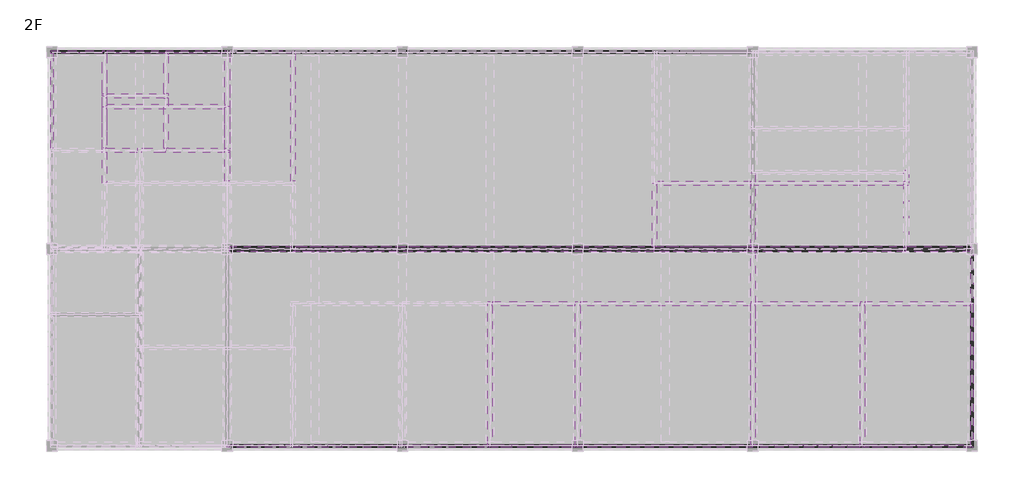
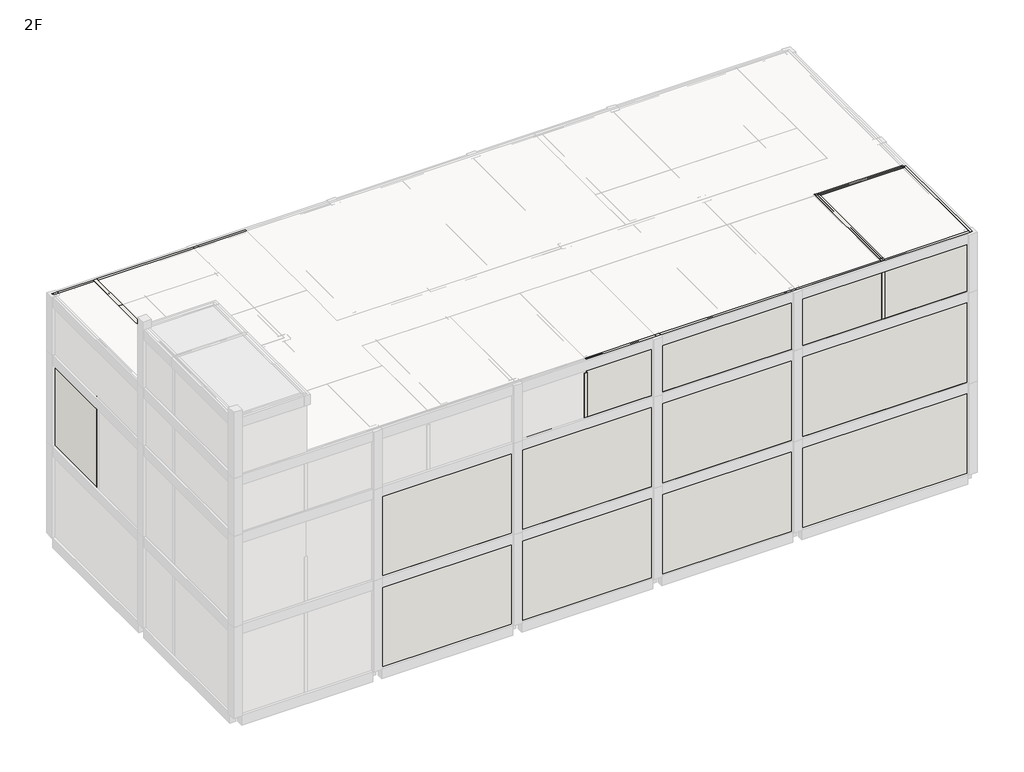
# One storey, part 2 of 7: 53 walls.
"""IFC4 building model written with IfcOpenShell, lengths in millimetres."""

from ifc_helpers import new_model, si_unit, frame, origin, place, context, project, spatial, polyline, outline, extrude, faceted_brep, element, save

model = new_model("IFC4")

# Units and contexts
model_context = context("Model", 3, world=origin())
ifc_project = project(units=[si_unit("LENGTHUNIT", "METRE", prefix="MILLI")], contexts=[model_context])

# Site, building, storey
site = spatial("IfcSite", under=ifc_project)
building = spatial("IfcBuilding", under=site)
storey = spatial("IfcBuildingStorey", under=building, Name="2F", Elevation=3500.0)

# Walls
placement = place(None, origin())
element("IfcWall", 1, ObjectType="WA211_Exterior-Cement Brick-90mm", at=placement, inside=storey, context=model_context, shape_type="Brep", body=[
    faceted_brep([(45402.6521483, 181866.8614395, 3500.0), (45516.6521483, 181866.8614395, 3500.0), (77352.6521483, 181866.8614395, 3500.0), (77352.6521483, 181866.8614395, 9000.0), (45516.6521483, 181866.8614395, 9000.0), (45402.6521483, 181866.8614395, 9000.0), (45402.6521483, 181980.8614395, 3500.0), (45402.6521483, 181980.8614395, 9000.0), (77352.6521483, 181980.8614395, 9000.0), (77352.6521483, 181980.8614395, 3500.0)], [[[0, 1, 2, 3, 4, 5]], [[6, 7, 8, 9]], [[2, 1, 0, 6, 9]], [[5, 4, 3, 8, 7]], [[0, 5, 7, 6]], [[3, 2, 9, 8]]]),
])
element("IfcWall", 2, ObjectType="WA211_Exterior-Cement Brick-90mm", at=placement, inside=storey, context=model_context, shape_type="SweptSolid", body=[
    extrude(outline(polyline([(53566.6521483, 163980.8614395), (87402.6521483, 163980.8614395), (87402.6521483, 163866.8614395), (53566.6521483, 163866.8614395), (53566.6521483, 163980.8614395)])), frame((0.0, 0.0, 3500.0), z_axis=(0.0, 0.0, 1.0), x_axis=(1.0, 0.0, 0.0)), (0.0, 0.0, 1.0), 5500.0),
])
element("IfcWall", 3, ObjectType="WA211_Exterior-Cement Brick-90mm", at=placement, inside=storey, context=model_context, shape_type="Brep", body=[
    faceted_brep([(87402.6521483, 172923.8614395, 3500.0), (87402.6521483, 172816.8614395, 3500.0), (87402.6521483, 163980.8614395, 3500.0), (87402.6521483, 163866.8614395, 3500.0), (87402.6521483, 163866.8614395, 9000.0), (87402.6521483, 163980.8614395, 9000.0), (87402.6521483, 172816.8614395, 9000.0), (87402.6521483, 172923.8614395, 9000.0), (87516.6521483, 172923.8614395, 3500.0), (87516.6521483, 172923.8614395, 9000.0), (87516.6521483, 163866.8614395, 9000.0), (87516.6521483, 163866.8614395, 3500.0)], [[[0, 1, 2, 3, 4, 5, 6, 7]], [[8, 9, 10, 11]], [[3, 2, 1, 0, 8, 11]], [[7, 6, 5, 4, 10, 9]], [[0, 7, 9, 8]], [[4, 3, 11, 10]]]),
])
element("IfcWall", 4, ObjectType="WA211_Exterior-Cement Brick-90mm", at=placement, inside=storey, context=model_context, shape_type="Brep", body=[
    faceted_brep([(77459.6521483, 163980.8614395, 9000.0), (77352.6521483, 163980.8614395, 9000.0), (53566.6521483, 163980.8614395, 9000.0), (53566.6521483, 163980.8614395, 12000.0), (53459.6521483, 163980.8614395, 12000.0), (53459.6521483, 163980.8614395, 14500.0), (77352.6521483, 163980.8614395, 14500.0), (77459.6521483, 163980.8614395, 14500.0), (77459.6521483, 163866.8614395, 9000.0), (77459.6521483, 163866.8614395, 14500.0), (53459.6521483, 163866.8614395, 14500.0), (53459.6521483, 163866.8614395, 12000.0), (53566.6521483, 163866.8614395, 12000.0), (53566.6521483, 163866.8614395, 9000.0)], [[[0, 1, 2, 3, 4, 5, 6, 7]], [[8, 9, 10, 11, 12, 13]], [[2, 1, 0, 8, 13]], [[7, 6, 5, 10, 9]], [[0, 7, 9, 8]], [[5, 4, 11, 10]], [[11, 4, 3, 12]], [[3, 2, 13, 12]]]),
])
element("IfcWall", 5, ObjectType="WA211_Exterior-Cement Brick-90mm", at=placement, inside=storey, context=model_context, shape_type="Brep", body=[
    faceted_brep([(87402.6521483, 163980.8614395, 9000.0), (77566.6521483, 163980.8614395, 9000.0), (77459.6521483, 163980.8614395, 9000.0), (77459.6521483, 163980.8614395, 14500.0), (77566.6521483, 163980.8614395, 14500.0), (87402.6521483, 163980.8614395, 14500.0), (87402.6521483, 163866.8614395, 9000.0), (87402.6521483, 163866.8614395, 14500.0), (77459.6521483, 163866.8614395, 14500.0), (77459.6521483, 163866.8614395, 9000.0)], [[[0, 1, 2, 3, 4, 5]], [[6, 7, 8, 9]], [[2, 1, 0, 6, 9]], [[3, 2, 9, 8]], [[5, 4, 3, 8, 7]], [[0, 5, 7, 6]]]),
])
element("IfcWall", 6, ObjectType="WA211_Exterior-Cement Brick-90mm", at=placement, inside=storey, context=model_context, shape_type="Brep", body=[
    faceted_brep([(87402.6521483, 172923.8614395, 9000.0), (87402.6521483, 172816.8614395, 9000.0), (87402.6521483, 163980.8614395, 9000.0), (87402.6521483, 163866.8614395, 9000.0), (87402.6521483, 163866.8614395, 14500.0), (87402.6521483, 163980.8614395, 14500.0), (87402.6521483, 172816.8614395, 14500.0), (87402.6521483, 172923.8614395, 14500.0), (87516.6521483, 172923.8614395, 9000.0), (87516.6521483, 172923.8614395, 14500.0), (87516.6521483, 163866.8614395, 14500.0), (87516.6521483, 163866.8614395, 9000.0)], [[[0, 1, 2, 3, 4, 5, 6, 7]], [[8, 9, 10, 11]], [[3, 2, 1, 0, 8, 11]], [[7, 6, 5, 4, 10, 9]], [[0, 7, 9, 8]], [[4, 3, 11, 10]]]),
])
element("IfcWall", 7, ObjectType="WA211_Exterior-Cement Brick-90mm", at=placement, inside=storey, context=model_context, shape_type="SweptSolid", body=[
    extrude(outline(polyline([(45516.6521483, 181866.8614395), (45516.6521483, 177530.8614395), (45402.6521483, 177530.8614395), (45402.6521483, 181866.8614395), (45516.6521483, 181866.8614395)])), frame((0.0, 0.0, 9000.0), z_axis=(0.0, 0.0, 1.0), x_axis=(1.0, 0.0, 0.0)), (0.0, 0.0, 1.0), 5500.0),
])
element("IfcWall", 8, ObjectType="WA211_Exterior-Cement Brick-90mm", at=placement, inside=storey, context=model_context, shape_type="Brep", body=[
    faceted_brep([(45402.6521483, 181866.8614395, 9000.0), (45516.6521483, 181866.8614395, 9000.0), (47752.6521483, 181866.8614395, 9000.0), (47752.6521483, 181866.8614395, 14500.0), (45516.6521483, 181866.8614395, 14500.0), (45402.6521483, 181866.8614395, 14500.0), (45402.6521483, 181980.8614395, 9000.0), (45402.6521483, 181980.8614395, 14500.0), (47752.6521483, 181980.8614395, 14500.0), (47752.6521483, 181980.8614395, 9000.0)], [[[0, 1, 2, 3, 4, 5]], [[6, 7, 8, 9]], [[2, 1, 0, 6, 9]], [[5, 4, 3, 8, 7]], [[0, 5, 7, 6]], [[3, 2, 9, 8]]]),
])
element("IfcWall", 9, ObjectType="WA211_Exterior-Cement Brick-90mm", at=placement, inside=storey, context=model_context, shape_type="Brep", body=[
    faceted_brep([(50659.6521483, 181866.8614395, 14500.0), (50659.6521483, 181866.8614395, 9000.0), (50766.6521483, 181866.8614395, 9000.0), (53352.6521483, 181866.8614395, 9000.0), (53352.6521483, 181866.8614395, 12400.0), (53459.6521483, 181866.8614395, 12400.0), (53459.6521483, 181866.8614395, 14500.0), (50659.6521483, 181980.8614395, 9000.0), (50659.6521483, 181980.8614395, 14500.0), (53459.6521483, 181980.8614395, 14500.0), (53459.6521483, 181980.8614395, 12400.0), (53352.6521483, 181980.8614395, 12400.0), (53352.6521483, 181980.8614395, 9000.0)], [[[0, 1, 2, 3, 4, 5, 6]], [[7, 8, 9, 10, 11, 12]], [[3, 2, 1, 7, 12]], [[0, 6, 9, 8]], [[6, 5, 10, 9]], [[10, 5, 4, 11]], [[4, 3, 12, 11]], [[0, 8, 7, 1]]]),
])
element("IfcWall", 10, ObjectType="WA211_Exterior-Cement Brick-90mm", at=placement, inside=storey, context=model_context, shape_type="Brep", body=[
    faceted_brep([(47966.6521483, 181866.8614395, 9000.0), (50552.6521483, 181866.8614395, 9000.0), (50659.6521483, 181866.8614395, 9000.0), (50659.6521483, 181866.8614395, 14500.0), (47966.6521483, 181866.8614395, 14500.0), (47966.6521483, 181980.8614395, 9000.0), (47966.6521483, 181980.8614395, 14500.0), (50659.6521483, 181980.8614395, 14500.0), (50659.6521483, 181980.8614395, 9000.0)], [[[0, 1, 2, 3, 4]], [[5, 6, 7, 8]], [[2, 1, 0, 5, 8]], [[4, 3, 7, 6]], [[0, 4, 6, 5]], [[2, 8, 7, 3]]]),
])
element("IfcWall", 11, ObjectType="WA211_Exterior-Cement Brick-90mm", at=placement, inside=storey, context=model_context, shape_type="SweptSolid", body=[
    extrude(outline(polyline([(14500.0, 69352.6521483), (17200.0, 69352.6521483), (17200.0, 69459.6521483), (18000.0, 69459.6521483), (18000.0, 65459.6521483), (17200.0, 65459.6521483), (17200.0, 65566.6521483), (14500.0, 65566.6521483), (14500.0, 69352.6521483)])), frame((0.0, 163866.8614395, 0.0), z_axis=(0.0, 1.0, 0.0), x_axis=(0.0, 0.0, 1.0)), (0.0, 0.0, 1.0), 114.0),
])
element("IfcWall", 12, ObjectType="WA211_Exterior-Cement Brick-90mm", at=placement, inside=storey, context=model_context, shape_type="Brep", body=[
    faceted_brep([(77459.6521483, 163980.8614395, 18000.0), (77459.6521483, 163980.8614395, 14500.0), (77352.6521483, 163980.8614395, 14500.0), (69566.6521483, 163980.8614395, 14500.0), (69566.6521483, 163980.8614395, 17200.0), (69459.6521483, 163980.8614395, 17200.0), (69459.6521483, 163980.8614395, 18000.0), (77459.6521483, 163866.8614395, 14500.0), (77459.6521483, 163866.8614395, 18000.0), (69459.6521483, 163866.8614395, 18000.0), (69459.6521483, 163866.8614395, 17200.0), (69566.6521483, 163866.8614395, 17200.0), (69566.6521483, 163866.8614395, 14500.0)], [[[0, 1, 2, 3, 4, 5, 6]], [[7, 8, 9, 10, 11, 12]], [[3, 2, 1, 7, 12]], [[0, 6, 9, 8]], [[6, 5, 10, 9]], [[10, 5, 4, 11]], [[4, 3, 12, 11]], [[0, 8, 7, 1]]]),
])
element("IfcWall", 13, ObjectType="WA211_Exterior-Cement Brick-90mm", at=placement, inside=storey, context=model_context, shape_type="Brep", body=[
    faceted_brep([(82352.6521483, 163980.8614395, 14500.0), (77566.6521483, 163980.8614395, 14500.0), (77459.6521483, 163980.8614395, 14500.0), (77459.6521483, 163980.8614395, 18000.0), (82352.6521483, 163980.8614395, 18000.0), (82352.6521483, 163866.8614395, 14500.0), (82352.6521483, 163866.8614395, 18000.0), (77459.6521483, 163866.8614395, 18000.0), (77459.6521483, 163866.8614395, 14500.0)], [[[0, 1, 2, 3, 4]], [[5, 6, 7, 8]], [[2, 1, 0, 5, 8]], [[4, 3, 7, 6]], [[2, 8, 7, 3]], [[0, 4, 6, 5]]]),
])
element("IfcWall", 14, ObjectType="WA211_Exterior-Cement Brick-90mm", at=placement, inside=storey, context=model_context, shape_type="SweptSolid", body=[
    extrude(outline(polyline([(82566.6521483, 163980.8614395), (87402.6521483, 163980.8614395), (87402.6521483, 163866.8614395), (82566.6521483, 163866.8614395), (82566.6521483, 163980.8614395)])), frame((0.0, 0.0, 14500.0), z_axis=(0.0, 0.0, 1.0), x_axis=(1.0, 0.0, 0.0)), (0.0, 0.0, 1.0), 3500.0),
])
element("IfcWall", 15, ObjectType="WA211_Exterior-Cement Brick-90mm", at=placement, inside=storey, context=model_context, shape_type="Brep", body=[
    faceted_brep([(87402.6521483, 170423.8614395, 14500.0), (87402.6521483, 170316.8614395, 14500.0), (87402.6521483, 163980.8614395, 14500.0), (87402.6521483, 163866.8614395, 14500.0), (87402.6521483, 163866.8614395, 18000.0), (87402.6521483, 163980.8614395, 18000.0), (87402.6521483, 170316.8614395, 18000.0), (87402.6521483, 170423.8614395, 18000.0), (87516.6521483, 170423.8614395, 14500.0), (87516.6521483, 170423.8614395, 18000.0), (87516.6521483, 163866.8614395, 18000.0), (87516.6521483, 163866.8614395, 14500.0)], [[[0, 1, 2, 3, 4, 5, 6, 7]], [[8, 9, 10, 11]], [[3, 2, 1, 0, 8, 11]], [[7, 6, 5, 4, 10, 9]], [[0, 7, 9, 8]], [[4, 3, 11, 10]]]),
])
element("IfcWall", 16, ObjectType="WA211_Exterior-Cement Brick-90mm", at=placement, inside=storey, context=model_context, shape_type="SweptSolid", body=[
    extrude(outline(polyline([(14500.0, 47966.6521483), (14500.0, 53352.6521483), (17200.0, 53352.6521483), (17200.0, 53459.6521483), (18000.0, 53459.6521483), (18000.0, 47966.6521483), (14500.0, 47966.6521483)])), frame((0.0, 181866.8614395, 0.0), z_axis=(0.0, 1.0, 0.0), x_axis=(0.0, 0.0, 1.0)), (0.0, 0.0, 1.0), 114.0),
])
element("IfcWall", 17, ObjectType="WA211_Exterior-Cement Brick-90mm", at=placement, inside=storey, context=model_context, shape_type="SweptSolid", body=[
    extrude(outline(polyline([(14500.0, 53566.6521483), (14500.0, 56352.6521483), (17200.0, 56352.6521483), (17200.0, 56459.6521483), (18000.0, 56459.6521483), (18000.0, 53459.6521483), (17200.0, 53459.6521483), (17200.0, 53566.6521483), (14500.0, 53566.6521483)])), frame((0.0, 181866.8614395, 0.0), z_axis=(0.0, 1.0, 0.0), x_axis=(0.0, 0.0, 1.0)), (0.0, 0.0, 1.0), 114.0),
])
element("IfcWall", 18, ObjectType="WA211_Exterior-Cement Brick-90mm", at=placement, inside=storey, context=model_context, shape_type="Brep", body=[
    faceted_brep([(45402.6521483, 181866.8614395, 14500.0), (45516.6521483, 181866.8614395, 14500.0), (47752.6521483, 181866.8614395, 14500.0), (47752.6521483, 181866.8614395, 18000.0), (45516.6521483, 181866.8614395, 18000.0), (45402.6521483, 181866.8614395, 18000.0), (45402.6521483, 181980.8614395, 14500.0), (45402.6521483, 181980.8614395, 18000.0), (47752.6521483, 181980.8614395, 18000.0), (47752.6521483, 181980.8614395, 14500.0)], [[[0, 1, 2, 3, 4, 5]], [[6, 7, 8, 9]], [[2, 1, 0, 6, 9]], [[5, 4, 3, 8, 7]], [[3, 2, 9, 8]], [[0, 5, 7, 6]]]),
])
element("IfcWall", 19, ObjectType="WA221_Interior-Cement Block-190mm", at=placement, inside=storey, context=model_context, shape_type="SweptSolid", body=[
    extrude(outline(polyline([(53566.6521483, 173030.8614395), (77352.6521483, 173030.8614395), (77352.6521483, 172816.8614395), (53566.6521483, 172816.8614395), (53566.6521483, 173030.8614395)])), frame((0.0, 0.0, 3500.0), z_axis=(0.0, 0.0, 1.0), x_axis=(1.0, 0.0, 0.0)), (0.0, 0.0, 1.0), 5500.0),
])
element("IfcWall", 20, ObjectType="WA221_Interior-Cement Block-190mm", at=placement, inside=storey, context=model_context, shape_type="Brep", body=[
    faceted_brep([(77566.6521483, 172816.8614395, 3500.0), (87402.6521483, 172816.8614395, 3500.0), (87402.6521483, 172816.8614395, 9000.0), (77566.6521483, 172816.8614395, 9000.0), (77566.6521483, 173030.8614395, 3500.0), (77566.6521483, 173030.8614395, 9000.0), (87402.6521483, 173030.8614395, 9000.0), (87402.6521483, 173030.8614395, 3500.0), (87402.6521483, 172923.8614395, 3500.0), (87402.6521483, 172923.8614395, 9000.0)], [[[0, 1, 2, 3]], [[4, 5, 6, 7]], [[1, 0, 4, 7, 8]], [[3, 2, 9, 6, 5]], [[0, 3, 5, 4]], [[2, 1, 8, 7, 6, 9]]]),
])
element("IfcWall", 21, ObjectType="WA221_Interior-Cement Block-190mm", at=placement, inside=storey, context=model_context, shape_type="Brep", body=[
    faceted_brep([(77459.6521483, 173030.8614395, 9000.0), (77352.6521483, 173030.8614395, 9000.0), (53566.6521483, 173030.8614395, 9000.0), (53566.6521483, 173030.8614395, 12400.0), (77352.6521483, 173030.8614395, 12400.0), (77459.6521483, 173030.8614395, 12400.0), (77459.6521483, 172816.8614395, 9000.0), (77459.6521483, 172816.8614395, 12400.0), (77352.6521483, 172816.8614395, 12400.0), (53566.6521483, 172816.8614395, 12400.0), (53566.6521483, 172816.8614395, 12000.0), (53566.6521483, 172816.8614395, 9000.0), (77352.6521483, 172816.8614395, 9000.0), (53566.6521483, 172923.8614395, 9000.0)], [[[0, 1, 2, 3, 4, 5]], [[6, 7, 8, 9, 10, 11, 12]], [[2, 1, 0, 6, 12, 11, 13]], [[5, 4, 3, 9, 8, 7]], [[0, 5, 7, 6]], [[2, 13, 11, 10, 9, 3]]]),
])
element("IfcWall", 22, ObjectType="WA221_Interior-Cement Block-190mm", at=placement, inside=storey, context=model_context, shape_type="Brep", body=[
    faceted_brep([(77352.6521483, 176316.8614395, 9000.0), (77352.6521483, 173030.8614395, 9000.0), (77352.6521483, 173030.8614395, 12400.0), (77352.6521483, 176423.8614395, 12400.0), (77352.6521483, 176423.8614395, 11700.0), (77352.6521483, 176316.8614395, 11700.0), (77566.6521483, 176316.8614395, 9000.0), (77566.6521483, 176316.8614395, 11700.0), (77566.6521483, 176423.8614395, 11700.0), (77566.6521483, 176423.8614395, 12400.0), (77566.6521483, 173030.8614395, 12400.0), (77566.6521483, 173030.8614395, 9000.0), (77459.6521483, 173030.8614395, 9000.0), (77459.6521483, 173030.8614395, 12400.0)], [[[0, 1, 2, 3, 4, 5]], [[6, 7, 8, 9, 10, 11]], [[1, 0, 6, 11, 12]], [[3, 2, 13, 10, 9]], [[2, 1, 12, 11, 10, 13]], [[4, 3, 9, 8]], [[4, 8, 7, 5]], [[0, 5, 7, 6]]]),
])
element("IfcWall", 23, ObjectType="WA221_Interior-Cement Block-190mm", at=placement, inside=storey, context=model_context, shape_type="Brep", body=[
    faceted_brep([(53566.6521483, 177530.8614395, 9000.0), (53566.6521483, 181866.8614395, 9000.0), (53566.6521483, 181980.8614395, 9000.0), (53566.6521483, 181980.8614395, 12400.0), (53566.6521483, 181866.8614395, 12400.0), (53566.6521483, 177423.8614395, 12400.0), (53566.6521483, 177423.8614395, 11700.0), (53566.6521483, 177530.8614395, 11700.0), (53352.6521483, 177530.8614395, 9000.0), (53352.6521483, 177530.8614395, 11700.0), (53352.6521483, 177423.8614395, 11700.0), (53352.6521483, 177423.8614395, 12400.0), (53352.6521483, 181866.8614395, 12400.0), (53352.6521483, 181980.8614395, 12400.0), (53352.6521483, 181980.8614395, 9000.0), (53352.6521483, 181866.8614395, 9000.0), (53459.6521483, 181980.8614395, 12400.0)], [[[0, 1, 2, 3, 4, 5, 6, 7]], [[8, 9, 10, 11, 12, 13, 14, 15]], [[2, 1, 0, 8, 15, 14]], [[5, 4, 3, 16, 13, 12, 11]], [[3, 2, 14, 13, 16]], [[6, 5, 11, 10]], [[6, 10, 9, 7]], [[0, 7, 9, 8]]]),
])
element("IfcWall", 24, ObjectType="WA221_Interior-Cement Block-190mm", at=placement, inside=storey, context=model_context, shape_type="Brep", body=[
    faceted_brep([(77566.6521483, 163980.8614395, 9000.0), (77566.6521483, 172816.8614395, 9000.0), (77566.6521483, 172816.8614395, 14500.0), (77566.6521483, 163980.8614395, 14500.0), (77352.6521483, 163980.8614395, 9000.0), (77352.6521483, 163980.8614395, 14500.0), (77352.6521483, 172816.8614395, 14500.0), (77352.6521483, 172816.8614395, 12400.0), (77352.6521483, 172816.8614395, 9000.0), (77459.6521483, 163980.8614395, 9000.0), (77459.6521483, 172816.8614395, 9000.0), (77459.6521483, 163980.8614395, 14500.0)], [[[0, 1, 2, 3]], [[4, 5, 6, 7, 8]], [[1, 0, 9, 4, 8, 10]], [[3, 2, 6, 5, 11]], [[1, 10, 8, 7, 6, 2]], [[0, 3, 11, 5, 4, 9]]]),
])
element("IfcWall", 25, ObjectType="WA221_Interior-Cement Block-190mm", at=placement, inside=storey, context=model_context, shape_type="Brep", body=[
    faceted_brep([(77459.6521483, 172816.8614395, 9000.0), (77566.6521483, 172816.8614395, 9000.0), (84459.6521483, 172816.8614395, 9000.0), (84459.6521483, 172816.8614395, 14500.0), (77566.6521483, 172816.8614395, 14500.0), (77352.6521483, 172816.8614395, 14500.0), (77352.6521483, 172816.8614395, 12400.0), (77459.6521483, 172816.8614395, 12400.0), (77459.6521483, 173030.8614395, 9000.0), (77459.6521483, 173030.8614395, 12400.0), (77352.6521483, 173030.8614395, 12400.0), (77352.6521483, 173030.8614395, 14500.0), (84459.6521483, 173030.8614395, 14500.0), (84459.6521483, 173030.8614395, 9000.0), (84352.6521483, 173030.8614395, 9000.0), (77566.6521483, 173030.8614395, 9000.0)], [[[0, 1, 2, 3, 4, 5, 6, 7]], [[8, 9, 10, 11, 12, 13, 14, 15]], [[2, 1, 0, 8, 15, 14, 13]], [[5, 4, 3, 12, 11]], [[0, 7, 9, 8]], [[6, 10, 9, 7]], [[6, 5, 11, 10]], [[2, 13, 12, 3]]]),
])
element("IfcWall", 26, ObjectType="WA221_Interior-Cement Block-190mm", at=placement, inside=storey, context=model_context, shape_type="Brep", body=[
    faceted_brep([(84459.6521483, 172816.8614395, 14500.0), (84459.6521483, 172816.8614395, 9000.0), (87402.6521483, 172816.8614395, 9000.0), (87402.6521483, 172816.8614395, 14500.0), (84459.6521483, 173030.8614395, 9000.0), (84459.6521483, 173030.8614395, 14500.0), (87402.6521483, 173030.8614395, 14500.0), (87402.6521483, 173030.8614395, 9000.0), (84566.6521483, 173030.8614395, 9000.0), (87402.6521483, 172923.8614395, 9000.0), (87402.6521483, 172923.8614395, 14500.0)], [[[0, 1, 2, 3]], [[4, 5, 6, 7, 8]], [[2, 1, 4, 8, 7, 9]], [[0, 3, 10, 6, 5]], [[3, 2, 9, 7, 6, 10]], [[0, 5, 4, 1]]]),
])
element("IfcWall", 27, ObjectType="WA221_Interior-Cement Block-190mm", at=placement, inside=storey, context=model_context, shape_type="Brep", body=[
    faceted_brep([(84352.6521483, 176530.8614395, 9000.0), (84352.6521483, 176316.8614395, 9000.0), (84352.6521483, 173030.8614395, 9000.0), (84352.6521483, 173030.8614395, 11700.0), (84352.6521483, 176316.8614395, 11700.0), (84352.6521483, 176530.8614395, 11700.0), (84566.6521483, 176530.8614395, 9000.0), (84566.6521483, 176530.8614395, 11700.0), (84566.6521483, 173030.8614395, 11700.0), (84566.6521483, 173030.8614395, 9000.0), (84459.6521483, 173030.8614395, 9000.0)], [[[0, 1, 2, 3, 4, 5]], [[6, 7, 8, 9]], [[2, 1, 0, 6, 9, 10]], [[5, 4, 3, 8, 7]], [[0, 5, 7, 6]], [[3, 2, 10, 9, 8]]]),
])
element("IfcWall", 28, ObjectType="WA221_Interior-Cement Block-190mm", at=placement, inside=storey, context=model_context, shape_type="Brep", body=[
    faceted_brep([(47752.6521483, 181980.8614395, 9000.0), (47752.6521483, 181866.8614395, 9000.0), (47752.6521483, 180030.8614395, 9000.0), (47752.6521483, 180030.8614395, 11700.0), (47752.6521483, 179923.8614395, 11700.0), (47752.6521483, 179923.8614395, 14500.0), (47752.6521483, 181866.8614395, 14500.0), (47752.6521483, 181980.8614395, 14500.0), (47966.6521483, 181980.8614395, 9000.0), (47966.6521483, 181980.8614395, 14500.0), (47966.6521483, 181866.8614395, 14500.0), (47966.6521483, 179923.8614395, 14500.0), (47966.6521483, 179923.8614395, 11700.0), (47966.6521483, 180030.8614395, 11700.0), (47966.6521483, 180030.8614395, 9000.0), (47966.6521483, 181866.8614395, 9000.0)], [[[0, 1, 2, 3, 4, 5, 6, 7]], [[8, 9, 10, 11, 12, 13, 14, 15]], [[2, 1, 0, 8, 15, 14]], [[7, 6, 5, 11, 10, 9]], [[0, 7, 9, 8]], [[5, 4, 12, 11]], [[12, 4, 3, 13]], [[3, 2, 14, 13]]]),
])
element("IfcWall", 29, ObjectType="WA221_Interior-Cement Block-190mm", at=placement, inside=storey, context=model_context, shape_type="Brep", body=[
    faceted_brep([(47752.6521483, 179816.8614395, 9000.0), (47752.6521483, 177530.8614395, 9000.0), (47752.6521483, 177530.8614395, 14500.0), (47752.6521483, 179923.8614395, 14500.0), (47752.6521483, 179923.8614395, 11700.0), (47752.6521483, 179816.8614395, 11700.0), (47966.6521483, 179816.8614395, 9000.0), (47966.6521483, 179816.8614395, 11700.0), (47966.6521483, 179923.8614395, 11700.0), (47966.6521483, 179923.8614395, 14500.0), (47966.6521483, 177530.8614395, 14500.0), (47966.6521483, 177530.8614395, 11700.0), (47966.6521483, 177530.8614395, 9000.0), (47859.6521483, 177530.8614395, 9000.0)], [[[0, 1, 2, 3, 4, 5]], [[6, 7, 8, 9, 10, 11, 12]], [[1, 0, 6, 12, 13]], [[3, 2, 10, 9]], [[1, 13, 12, 11, 10, 2]], [[4, 3, 9, 8]], [[4, 8, 7, 5]], [[0, 5, 7, 6]]]),
])
element("IfcWall", 30, ObjectType="WA221_Interior-Cement Block-190mm", at=placement, inside=storey, context=model_context, shape_type="Brep", body=[
    faceted_brep([(49352.6521483, 177530.8614395, 9000.0), (47966.6521483, 177530.8614395, 9000.0), (47859.6521483, 177530.8614395, 9000.0), (47859.6521483, 177530.8614395, 11700.0), (47966.6521483, 177530.8614395, 11700.0), (49352.6521483, 177530.8614395, 11700.0), (49352.6521483, 177316.8614395, 9000.0), (49352.6521483, 177316.8614395, 11700.0), (47966.6521483, 177316.8614395, 11700.0), (47859.6521483, 177316.8614395, 11700.0), (47859.6521483, 177316.8614395, 9000.0)], [[[0, 1, 2, 3, 4, 5]], [[6, 7, 8, 9, 10]], [[2, 1, 0, 6, 10]], [[3, 2, 10, 9]], [[5, 4, 3, 9, 8, 7]], [[0, 5, 7, 6]]]),
])
element("IfcWall", 31, ObjectType="WA221_Interior-Cement Block-190mm", at=placement, inside=storey, context=model_context, shape_type="Brep", body=[
    faceted_brep([(50552.6521483, 181866.8614395, 9000.0), (50552.6521483, 180030.8614395, 9000.0), (50552.6521483, 180030.8614395, 11700.0), (50552.6521483, 181866.8614395, 11700.0), (50766.6521483, 181866.8614395, 9000.0), (50766.6521483, 181866.8614395, 11700.0), (50766.6521483, 180030.8614395, 11700.0), (50766.6521483, 180030.8614395, 9000.0), (50659.6521483, 181866.8614395, 9000.0)], [[[0, 1, 2, 3]], [[4, 5, 6, 7]], [[1, 0, 8, 4, 7]], [[3, 2, 6, 5]], [[0, 3, 5, 4, 8]], [[2, 1, 7, 6]]]),
])
element("IfcWall", 32, ObjectType="WA221_Interior-Cement Block-190mm", at=placement, inside=storey, context=model_context, shape_type="Brep", body=[
    faceted_brep([(50766.6521483, 177530.8614395, 9000.0), (50766.6521483, 179816.8614395, 9000.0), (50766.6521483, 179816.8614395, 11700.0), (50766.6521483, 177530.8614395, 11700.0), (50552.6521483, 177530.8614395, 9000.0), (50552.6521483, 177530.8614395, 11700.0), (50552.6521483, 179816.8614395, 11700.0), (50552.6521483, 179816.8614395, 9000.0), (50659.6521483, 177530.8614395, 9000.0), (50659.6521483, 177530.8614395, 11700.0)], [[[0, 1, 2, 3]], [[4, 5, 6, 7]], [[1, 0, 8, 4, 7]], [[3, 2, 6, 5, 9]], [[0, 3, 9, 5, 4, 8]], [[2, 1, 7, 6]]]),
])
element("IfcWall", 33, ObjectType="WA221_Interior-Cement Block-190mm", at=placement, inside=storey, context=model_context, shape_type="Brep", body=[
    faceted_brep([(50659.6521483, 177316.8614395, 9000.0), (53352.6521483, 177316.8614395, 9000.0), (53566.6521483, 177316.8614395, 9000.0), (53566.6521483, 177316.8614395, 11700.0), (53352.6521483, 177316.8614395, 11700.0), (50659.6521483, 177316.8614395, 11700.0), (50659.6521483, 177530.8614395, 9000.0), (50659.6521483, 177530.8614395, 11700.0), (50766.6521483, 177530.8614395, 11700.0), (53352.6521483, 177530.8614395, 11700.0), (53566.6521483, 177530.8614395, 11700.0), (53566.6521483, 177530.8614395, 9000.0), (53352.6521483, 177530.8614395, 9000.0), (50766.6521483, 177530.8614395, 9000.0), (53566.6521483, 177423.8614395, 11700.0)], [[[0, 1, 2, 3, 4, 5]], [[6, 7, 8, 9, 10, 11, 12, 13]], [[2, 1, 0, 6, 13, 12, 11]], [[5, 4, 3, 14, 10, 9, 8, 7]], [[0, 5, 7, 6]], [[3, 2, 11, 10, 14]]]),
])
element("IfcWall", 34, ObjectType="WA221_Interior-Cement Block-190mm", at=placement, inside=storey, context=model_context, shape_type="Brep", body=[
    faceted_brep([(50766.6521483, 180030.8614395, 9000.0), (50552.6521483, 180030.8614395, 9000.0), (47966.6521483, 180030.8614395, 9000.0), (47752.6521483, 180030.8614395, 9000.0), (47752.6521483, 180030.8614395, 11700.0), (47966.6521483, 180030.8614395, 11700.0), (50552.6521483, 180030.8614395, 11700.0), (50766.6521483, 180030.8614395, 11700.0), (50766.6521483, 179816.8614395, 9000.0), (50766.6521483, 179816.8614395, 11700.0), (50552.6521483, 179816.8614395, 11700.0), (47966.6521483, 179816.8614395, 11700.0), (47752.6521483, 179816.8614395, 11700.0), (47752.6521483, 179816.8614395, 9000.0), (47966.6521483, 179816.8614395, 9000.0), (50552.6521483, 179816.8614395, 9000.0), (47752.6521483, 179923.8614395, 11700.0)], [[[0, 1, 2, 3, 4, 5, 6, 7]], [[8, 9, 10, 11, 12, 13, 14, 15]], [[3, 2, 1, 0, 8, 15, 14, 13]], [[7, 6, 5, 4, 16, 12, 11, 10, 9]], [[0, 7, 9, 8]], [[4, 3, 13, 12, 16]]]),
])
element("IfcWall", 35, ObjectType="WA221_Interior-Cement Block-190mm", at=placement, inside=storey, context=model_context, shape_type="Brep", body=[
    faceted_brep([(50659.6521483, 177530.8614395, 9000.0), (50552.6521483, 177530.8614395, 9000.0), (49566.6521483, 177530.8614395, 9000.0), (49566.6521483, 177530.8614395, 11700.0), (50552.6521483, 177530.8614395, 11700.0), (50659.6521483, 177530.8614395, 11700.0), (50659.6521483, 177316.8614395, 9000.0), (50659.6521483, 177316.8614395, 11700.0), (49566.6521483, 177316.8614395, 11700.0), (49566.6521483, 177316.8614395, 9000.0)], [[[0, 1, 2, 3, 4, 5]], [[6, 7, 8, 9]], [[2, 1, 0, 6, 9]], [[5, 4, 3, 8, 7]], [[0, 5, 7, 6]], [[3, 2, 9, 8]]]),
])
element("IfcWall", 36, ObjectType="WA221_Interior-Cement Block-190mm", at=placement, inside=storey, context=model_context, shape_type="Brep", body=[
    faceted_brep([(65352.6521483, 170530.8614395, 14500.0), (65352.6521483, 170316.8614395, 14500.0), (65352.6521483, 163980.8614395, 14500.0), (65352.6521483, 163866.8614395, 14500.0), (65352.6521483, 163866.8614395, 17200.0), (65352.6521483, 163980.8614395, 17200.0), (65352.6521483, 170316.8614395, 17200.0), (65352.6521483, 170530.8614395, 17200.0), (65566.6521483, 170530.8614395, 14500.0), (65566.6521483, 170530.8614395, 17200.0), (65566.6521483, 170316.8614395, 17200.0), (65566.6521483, 163980.8614395, 17200.0), (65566.6521483, 163866.8614395, 17200.0), (65566.6521483, 163866.8614395, 14500.0), (65566.6521483, 163980.8614395, 14500.0), (65566.6521483, 170316.8614395, 14500.0), (65459.6521483, 163866.8614395, 17200.0)], [[[0, 1, 2, 3, 4, 5, 6, 7]], [[8, 9, 10, 11, 12, 13, 14, 15]], [[3, 2, 1, 0, 8, 15, 14, 13]], [[7, 6, 5, 4, 16, 12, 11, 10, 9]], [[4, 3, 13, 12, 16]], [[0, 7, 9, 8]]]),
])
element("IfcWall", 37, ObjectType="WA221_Interior-Cement Block-190mm", at=placement, inside=storey, context=model_context, shape_type="Brep", body=[
    faceted_brep([(69566.6521483, 163866.8614395, 14500.0), (69566.6521483, 163980.8614395, 14500.0), (69566.6521483, 170316.8614395, 14500.0), (69566.6521483, 170530.8614395, 14500.0), (69566.6521483, 170530.8614395, 17200.0), (69566.6521483, 170316.8614395, 17200.0), (69566.6521483, 163980.8614395, 17200.0), (69566.6521483, 163866.8614395, 17200.0), (69352.6521483, 163866.8614395, 14500.0), (69352.6521483, 163866.8614395, 17200.0), (69352.6521483, 163980.8614395, 17200.0), (69352.6521483, 170316.8614395, 17200.0), (69352.6521483, 170530.8614395, 17200.0), (69352.6521483, 170530.8614395, 14500.0), (69352.6521483, 170316.8614395, 14500.0), (69352.6521483, 163980.8614395, 14500.0), (69459.6521483, 163866.8614395, 17200.0)], [[[0, 1, 2, 3, 4, 5, 6, 7]], [[8, 9, 10, 11, 12, 13, 14, 15]], [[3, 2, 1, 0, 8, 15, 14, 13]], [[7, 6, 5, 4, 12, 11, 10, 9, 16]], [[4, 3, 13, 12]], [[0, 7, 16, 9, 8]]]),
])
element("IfcWall", 38, ObjectType="WA221_Interior-Cement Block-190mm", at=placement, inside=storey, context=model_context, shape_type="SweptSolid", body=[
    extrude(outline(polyline([(65566.6521483, 170530.8614395), (69352.6521483, 170530.8614395), (69352.6521483, 170316.8614395), (65566.6521483, 170316.8614395), (65566.6521483, 170530.8614395)])), frame((0.0, 0.0, 14500.0), z_axis=(0.0, 0.0, 1.0), x_axis=(1.0, 0.0, 0.0)), (0.0, 0.0, 1.0), 2700.0),
])
element("IfcWall", 39, ObjectType="WA221_Interior-Cement Block-190mm", at=placement, inside=storey, context=model_context, shape_type="Brep", body=[
    faceted_brep([(84566.6521483, 176030.8614395, 14500.0), (84352.6521483, 176030.8614395, 14500.0), (73066.6521483, 176030.8614395, 14500.0), (73066.6521483, 176030.8614395, 17200.0), (84352.6521483, 176030.8614395, 17200.0), (84566.6521483, 176030.8614395, 17200.0), (84566.6521483, 175816.8614395, 14500.0), (84566.6521483, 175816.8614395, 17200.0), (84352.6521483, 175816.8614395, 17200.0), (73066.6521483, 175816.8614395, 17200.0), (73066.6521483, 175816.8614395, 14500.0), (84352.6521483, 175816.8614395, 14500.0), (73066.6521483, 175923.8614395, 14500.0), (73066.6521483, 175923.8614395, 17200.0)], [[[0, 1, 2, 3, 4, 5]], [[6, 7, 8, 9, 10, 11]], [[2, 1, 0, 6, 11, 10, 12]], [[5, 4, 3, 13, 9, 8, 7]], [[0, 5, 7, 6]], [[3, 2, 12, 10, 9, 13]]]),
])
element("IfcWall", 40, ObjectType="WA221_Interior-Cement Block-190mm", at=placement, inside=storey, context=model_context, shape_type="Brep", body=[
    faceted_brep([(77352.6521483, 170530.8614395, 14500.0), (77352.6521483, 170316.8614395, 14500.0), (77352.6521483, 163980.8614395, 14500.0), (77352.6521483, 163980.8614395, 17200.0), (77352.6521483, 170316.8614395, 17200.0), (77352.6521483, 170530.8614395, 17200.0), (77566.6521483, 170530.8614395, 14500.0), (77566.6521483, 170530.8614395, 17200.0), (77566.6521483, 170316.8614395, 17200.0), (77566.6521483, 163980.8614395, 17200.0), (77566.6521483, 163980.8614395, 14500.0), (77566.6521483, 170316.8614395, 14500.0), (77459.6521483, 163980.8614395, 14500.0)], [[[0, 1, 2, 3, 4, 5]], [[6, 7, 8, 9, 10, 11]], [[2, 1, 0, 6, 11, 10, 12]], [[5, 4, 3, 9, 8, 7]], [[0, 5, 7, 6]], [[3, 2, 12, 10, 9]]]),
])
element("IfcWall", 41, ObjectType="WA221_Interior-Cement Block-190mm", at=placement, inside=storey, context=model_context, shape_type="SweptSolid", body=[
    extrude(outline(polyline([(77352.6521483, 170316.8614395), (69566.6521483, 170316.8614395), (69566.6521483, 170530.8614395), (77352.6521483, 170530.8614395), (77352.6521483, 170316.8614395)])), frame((0.0, 0.0, 14500.0), z_axis=(0.0, 0.0, 1.0), x_axis=(1.0, 0.0, 0.0)), (0.0, 0.0, 1.0), 2700.0),
])
element("IfcWall", 42, ObjectType="WA221_Interior-Cement Block-190mm", at=placement, inside=storey, context=model_context, shape_type="Brep", body=[
    faceted_brep([(73066.6521483, 173030.8614395, 14500.0), (73066.6521483, 175816.8614395, 14500.0), (73066.6521483, 175923.8614395, 14500.0), (73066.6521483, 175923.8614395, 17200.0), (73066.6521483, 175816.8614395, 17200.0), (73066.6521483, 173030.8614395, 17200.0), (72852.6521483, 173030.8614395, 14500.0), (72852.6521483, 173030.8614395, 17200.0), (72852.6521483, 175923.8614395, 17200.0), (72852.6521483, 175923.8614395, 14500.0), (72959.6521483, 173030.8614395, 14500.0), (72959.6521483, 173030.8614395, 17200.0)], [[[0, 1, 2, 3, 4, 5]], [[6, 7, 8, 9]], [[2, 1, 0, 10, 6, 9]], [[3, 2, 9, 8]], [[5, 4, 3, 8, 7, 11]], [[0, 5, 11, 7, 6, 10]]]),
])
element("IfcWall", 43, ObjectType="WA221_Interior-Cement Block-190mm", at=placement, inside=storey, context=model_context, shape_type="Brep", body=[
    faceted_brep([(56352.6521483, 181980.8614395, 14500.0), (56352.6521483, 181866.8614395, 14500.0), (56352.6521483, 176030.8614395, 14500.0), (56352.6521483, 176030.8614395, 17200.0), (56352.6521483, 181866.8614395, 17200.0), (56352.6521483, 181980.8614395, 17200.0), (56566.6521483, 181980.8614395, 14500.0), (56566.6521483, 181980.8614395, 17200.0), (56566.6521483, 181866.8614395, 17200.0), (56566.6521483, 176030.8614395, 17200.0), (56566.6521483, 176030.8614395, 14500.0), (56566.6521483, 181866.8614395, 14500.0), (56459.6521483, 181980.8614395, 17200.0)], [[[0, 1, 2, 3, 4, 5]], [[6, 7, 8, 9, 10, 11]], [[2, 1, 0, 6, 11, 10]], [[5, 4, 3, 9, 8, 7, 12]], [[0, 5, 12, 7, 6]], [[3, 2, 10, 9]]]),
])
element("IfcWall", 44, ObjectType="WA221_Interior-Cement Block-190mm", at=placement, inside=storey, context=model_context, shape_type="Brep", body=[
    faceted_brep([(72959.6521483, 173030.8614395, 14500.0), (72852.6521483, 173030.8614395, 14500.0), (56566.6521483, 173030.8614395, 14500.0), (56566.6521483, 173030.8614395, 17200.0), (72852.6521483, 173030.8614395, 17200.0), (72959.6521483, 173030.8614395, 17200.0), (72959.6521483, 172816.8614395, 14500.0), (72959.6521483, 172816.8614395, 17200.0), (56566.6521483, 172816.8614395, 17200.0), (56566.6521483, 172816.8614395, 14500.0)], [[[0, 1, 2, 3, 4, 5]], [[6, 7, 8, 9]], [[2, 1, 0, 6, 9]], [[5, 4, 3, 8, 7]], [[0, 5, 7, 6]], [[3, 2, 9, 8]]]),
])
element("IfcWall", 45, ObjectType="WA221_Interior-Cement Block-190mm", at=placement, inside=storey, context=model_context, shape_type="Brep", body=[
    faceted_brep([(82566.6521483, 163866.8614395, 14500.0), (82566.6521483, 163980.8614395, 14500.0), (82566.6521483, 170316.8614395, 14500.0), (82566.6521483, 170530.8614395, 14500.0), (82566.6521483, 170530.8614395, 18000.0), (82566.6521483, 170316.8614395, 18000.0), (82566.6521483, 163980.8614395, 18000.0), (82566.6521483, 163866.8614395, 18000.0), (82352.6521483, 163866.8614395, 14500.0), (82352.6521483, 163866.8614395, 18000.0), (82352.6521483, 163980.8614395, 18000.0), (82352.6521483, 170530.8614395, 18000.0), (82352.6521483, 170530.8614395, 17200.0), (82352.6521483, 170530.8614395, 14500.0), (82352.6521483, 170316.8614395, 14500.0), (82352.6521483, 163980.8614395, 14500.0)], [[[0, 1, 2, 3, 4, 5, 6, 7]], [[8, 9, 10, 11, 12, 13, 14, 15]], [[3, 2, 1, 0, 8, 15, 14, 13]], [[7, 6, 5, 4, 11, 10, 9]], [[3, 13, 12, 11, 4]], [[0, 7, 9, 8]]]),
])
element("IfcWall", 46, ObjectType="WA221_Interior-Cement Block-190mm", at=placement, inside=storey, context=model_context, shape_type="SweptSolid", body=[
    extrude(outline(polyline([(82352.6521483, 170316.8614395), (77566.6521483, 170316.8614395), (77566.6521483, 170530.8614395), (82352.6521483, 170530.8614395), (82352.6521483, 170316.8614395)])), frame((0.0, 0.0, 14500.0), z_axis=(0.0, 0.0, 1.0), x_axis=(1.0, 0.0, 0.0)), (0.0, 0.0, 1.0), 2700.0),
])
element("IfcWall", 47, ObjectType="WA221_Interior-Cement Block-190mm", at=placement, inside=storey, context=model_context, shape_type="Brep", body=[
    faceted_brep([(82566.6521483, 170316.8614395, 18000.0), (82566.6521483, 170316.8614395, 14500.0), (87402.6521483, 170316.8614395, 14500.0), (87402.6521483, 170316.8614395, 18000.0), (82566.6521483, 170530.8614395, 14500.0), (82566.6521483, 170530.8614395, 18000.0), (87402.6521483, 170530.8614395, 18000.0), (87402.6521483, 170530.8614395, 14500.0), (87402.6521483, 170423.8614395, 14500.0), (87402.6521483, 170423.8614395, 18000.0)], [[[0, 1, 2, 3]], [[4, 5, 6, 7]], [[2, 1, 4, 7, 8]], [[0, 3, 9, 6, 5]], [[0, 5, 4, 1]], [[3, 2, 8, 7, 6, 9]]]),
])
element("IfcWall", 48, ObjectType="WA221_Interior-Cement Block-190mm", at=placement, inside=storey, context=model_context, shape_type="Brep", body=[
    faceted_brep([(84352.6521483, 173030.8614395, 14500.0), (73066.6521483, 173030.8614395, 14500.0), (72959.6521483, 173030.8614395, 14500.0), (72959.6521483, 173030.8614395, 17200.0), (73066.6521483, 173030.8614395, 17200.0), (84352.6521483, 173030.8614395, 17200.0), (84352.6521483, 172816.8614395, 14500.0), (84352.6521483, 172816.8614395, 17200.0), (72959.6521483, 172816.8614395, 17200.0), (72959.6521483, 172816.8614395, 14500.0)], [[[0, 1, 2, 3, 4, 5]], [[6, 7, 8, 9]], [[2, 1, 0, 6, 9]], [[3, 2, 9, 8]], [[5, 4, 3, 8, 7]], [[0, 5, 7, 6]]]),
])
element("IfcWall", 49, ObjectType="WA221_Interior-Cement Block-190mm", at=placement, inside=storey, context=model_context, shape_type="Brep", body=[
    faceted_brep([(53352.6521483, 179530.8614395, 14500.0), (47966.6521483, 179530.8614395, 14500.0), (47966.6521483, 179530.8614395, 17200.0), (53352.6521483, 179530.8614395, 17200.0), (53352.6521483, 179316.8614395, 14500.0), (53352.6521483, 179316.8614395, 17200.0), (47966.6521483, 179316.8614395, 17200.0), (47966.6521483, 179316.8614395, 14500.0), (53352.6521483, 179423.8614395, 14500.0), (47966.6521483, 179423.8614395, 14500.0), (53352.6521483, 179423.8614395, 17200.0)], [[[0, 1, 2, 3]], [[4, 5, 6, 7]], [[1, 0, 8, 4, 7, 9]], [[3, 2, 6, 5, 10]], [[0, 3, 10, 5, 4, 8]], [[2, 1, 9, 7, 6]]]),
])
element("IfcWall", 50, ObjectType="WA221_Interior-Cement Block-190mm", at=placement, inside=storey, context=model_context, shape_type="Brep", body=[
    faceted_brep([(53352.6521483, 179423.8614395, 14500.0), (53352.6521483, 179316.8614395, 14500.0), (53352.6521483, 176030.8614395, 14500.0), (53352.6521483, 176030.8614395, 17200.0), (53352.6521483, 179316.8614395, 17200.0), (53352.6521483, 179423.8614395, 17200.0), (53566.6521483, 179423.8614395, 14500.0), (53566.6521483, 179423.8614395, 17200.0), (53566.6521483, 176030.8614395, 17200.0), (53566.6521483, 176030.8614395, 14500.0), (53459.6521483, 176030.8614395, 14500.0), (53459.6521483, 176030.8614395, 17200.0)], [[[0, 1, 2, 3, 4, 5]], [[6, 7, 8, 9]], [[2, 1, 0, 6, 9, 10]], [[5, 4, 3, 11, 8, 7]], [[0, 5, 7, 6]], [[3, 2, 10, 9, 8, 11]]]),
])
element("IfcWall", 51, ObjectType="WA221_Interior-Cement Block-190mm", at=placement, inside=storey, context=model_context, shape_type="Brep", body=[
    faceted_brep([(47752.6521483, 179423.8614395, 18000.0), (47752.6521483, 179423.8614395, 14500.0), (47752.6521483, 175923.8614395, 14500.0), (47752.6521483, 175923.8614395, 18000.0), (47966.6521483, 179423.8614395, 14500.0), (47966.6521483, 179423.8614395, 18000.0), (47966.6521483, 175923.8614395, 18000.0), (47966.6521483, 175923.8614395, 14500.0), (47966.6521483, 176030.8614395, 14500.0), (47966.6521483, 179316.8614395, 14500.0)], [[[0, 1, 2, 3]], [[4, 5, 6, 7, 8, 9]], [[2, 1, 4, 9, 8, 7]], [[0, 3, 6, 5]], [[0, 5, 4, 1]], [[2, 7, 6, 3]]]),
])
element("IfcWall", 52, ObjectType="WA221_Interior-Cement Block-190mm", at=placement, inside=storey, context=model_context, shape_type="Brep", body=[
    faceted_brep([(53352.6521483, 181980.8614395, 14500.0), (53352.6521483, 181866.8614395, 14500.0), (53352.6521483, 179530.8614395, 14500.0), (53352.6521483, 179423.8614395, 14500.0), (53352.6521483, 179423.8614395, 17200.0), (53352.6521483, 179530.8614395, 17200.0), (53352.6521483, 181866.8614395, 17200.0), (53352.6521483, 181980.8614395, 17200.0), (53566.6521483, 181980.8614395, 14500.0), (53566.6521483, 181980.8614395, 17200.0), (53566.6521483, 181866.8614395, 17200.0), (53566.6521483, 179423.8614395, 17200.0), (53566.6521483, 179423.8614395, 14500.0), (53566.6521483, 181866.8614395, 14500.0), (53459.6521483, 181980.8614395, 17200.0)], [[[0, 1, 2, 3, 4, 5, 6, 7]], [[8, 9, 10, 11, 12, 13]], [[3, 2, 1, 0, 8, 13, 12]], [[4, 3, 12, 11]], [[7, 6, 5, 4, 11, 10, 9, 14]], [[0, 7, 14, 9, 8]]]),
])
element("IfcWall", 53, ObjectType="WA221_Interior-Cement Block-190mm", at=placement, inside=storey, context=model_context, shape_type="Brep", body=[
    faceted_brep([(47752.6521483, 181980.8614395, 14500.0), (47752.6521483, 181866.8614395, 14500.0), (47752.6521483, 179423.8614395, 14500.0), (47752.6521483, 179423.8614395, 18000.0), (47752.6521483, 181866.8614395, 18000.0), (47752.6521483, 181980.8614395, 18000.0), (47966.6521483, 181980.8614395, 14500.0), (47966.6521483, 181980.8614395, 18000.0), (47966.6521483, 181866.8614395, 18000.0), (47966.6521483, 179423.8614395, 18000.0), (47966.6521483, 179423.8614395, 14500.0), (47966.6521483, 179530.8614395, 14500.0), (47966.6521483, 181866.8614395, 14500.0)], [[[0, 1, 2, 3, 4, 5]], [[6, 7, 8, 9, 10, 11, 12]], [[2, 1, 0, 6, 12, 11, 10]], [[5, 4, 3, 9, 8, 7]], [[2, 10, 9, 3]], [[0, 5, 7, 6]]]),
])

save(model, "model.ifc")

# Revit data of these elements
# Type "WA211_Exterior-Cement Brick-90mm"
#   Type Comments = ""
#   Layers, outside or top first: 0 mm "A04AL081-00001_Skirt_Acrylic Emulsion Paint" (function 100); 0 mm "A04AL077-00001_Ext Wall Painting_Acrylic Emulsion Paint" (function 100); 12 mm "A04AS164-00001_Plastering_Ext" (function 4); 90 mm "A04AK073-00001_Concrete Brick_0.5B" (function 1); 12 mm "A04AS164-00002_Plastering_Int" (function 5); 0 mm "A04AL078-00002_Int Wall Painting_Water Emulsion Paint" (function 100); 0 mm "A04AL081-00001_Skirt_Acrylic Emulsion Paint" (function 100)
# Type "WA221_Interior-Cement Block-190mm"
#   Type Comments = ""
#   Layers, outside or top first: 0 mm "A04AL081-00001_Skirt_Acrylic Emulsion Paint" (function 100); 0 mm "A04AL078-00002_Int Wall Painting_Water Emulsion Paint" (function 100); 12 mm "A04AS164-00002_Plastering_Int" (function 2); 190 mm "A04AK069-00002_Reinforced Concrete Block_THK 100-200mm" (function 1); 12 mm "A04AS164-00002_Plastering_Int" (function 2); 0 mm "A04AL078-00002_Int Wall Painting_Water Emulsion Paint" (function 100); 0 mm "A04AL081-00001_Skirt_Acrylic Emulsion Paint" (function 100)
# Elements 1, 3 (IfcWall, "WA211_Exterior-Cement Brick-90mm")
#   Top Offset = 0 mm
#   Base Offset = 0 mm
#   Unconnected Height = 5500 mm
#   wall height = 5500 mm
#   Phase Created = New Construction
#   Base Constraint = 2F
#   Materials on its faces: "Default Wall", "A04AS164-00001_Plastering_Ext", "A04AS164-00002_Plastering_Int"
# Element 2 (IfcWall, "WA211_Exterior-Cement Brick-90mm")
#   Top Offset = 0 mm
#   Base Offset = 0 mm
#   Unconnected Height = 5500 mm
#   wall height = 5500 mm
#   Phase Created = New Construction
#   Base Constraint = 2F
#   Materials on its faces: "Default Wall", "A04AS164-00002_Plastering_Int", "A04AS164-00001_Plastering_Ext"
# Elements 4, 5, 7, 9, 10 (IfcWall, "WA211_Exterior-Cement Brick-90mm")
#   Top Offset = 0 mm
#   Base Offset = 0 mm
#   Unconnected Height = 5500 mm
#   wall height = 5500 mm
#   Phase Created = New Construction
#   Base Constraint = 3F
#   Materials on its faces: "Default Wall", "A04AS164-00002_Plastering_Int", "A04AS164-00001_Plastering_Ext"
# Elements 6, 8 (IfcWall, "WA211_Exterior-Cement Brick-90mm")
#   Top Offset = 0 mm
#   Base Offset = 0 mm
#   Unconnected Height = 5500 mm
#   wall height = 5500 mm
#   Phase Created = New Construction
#   Base Constraint = 3F
#   Materials on its faces: "Default Wall", "A04AS164-00001_Plastering_Ext", "A04AS164-00002_Plastering_Int"
# Elements 11, 12, 13, 14, 16, 17 (IfcWall, "WA211_Exterior-Cement Brick-90mm")
#   Top Offset = 0 mm
#   Base Offset = 0 mm
#   Unconnected Height = 3500 mm
#   wall height = 3500 mm
#   Phase Created = New Construction
#   Base Constraint = 4F
#   Materials on its faces: "Default Wall", "A04AS164-00002_Plastering_Int", "A04AS164-00001_Plastering_Ext"
# Elements 15, 18 (IfcWall, "WA211_Exterior-Cement Brick-90mm")
#   Top Offset = 0 mm
#   Base Offset = 0 mm
#   Unconnected Height = 3500 mm
#   wall height = 3500 mm
#   Phase Created = New Construction
#   Base Constraint = 4F
#   Materials on its faces: "Default Wall", "A04AS164-00001_Plastering_Ext", "A04AS164-00002_Plastering_Int"
# Elements 19, 20 (IfcWall, "WA221_Interior-Cement Block-190mm")
#   Top Offset = 0 mm
#   Base Offset = 0 mm
#   Unconnected Height = 5500 mm
#   wall height = 5500 mm
#   Phase Created = New Construction
#   Base Constraint = 2F
#   Materials on its faces: "Default Wall", "A04AS164-00002_Plastering_Int"
# Elements 21, 22 (IfcWall, "WA221_Interior-Cement Block-190mm")
#   Top Offset = 0 mm
#   Base Offset = 0 mm
#   Unconnected Height = 3400 mm
#   wall height = 3400 mm
#   Phase Created = New Construction
#   Base Constraint = 3F
#   Materials on its faces: "Default Wall", "A04AS164-00002_Plastering_Int"
# Element 23 (IfcWall, "WA221_Interior-Cement Block-190mm")
#   Top Offset = 0 mm
#   Base Offset = 0 mm
#   Unconnected Height = 3400 mm
#   wall height = 3400 mm
#   Phase Created = New Construction
#   Base Constraint = 3F
#   Materials on its faces: "Default Wall", "A04AS164-00002_Plastering_Int", "A04AS164-00001_Plastering_Ext"
# Elements 24, 25, 26, 29 (IfcWall, "WA221_Interior-Cement Block-190mm")
#   Top Offset = 0 mm
#   Base Offset = 0 mm
#   Unconnected Height = 5500 mm
#   wall height = 5500 mm
#   Phase Created = New Construction
#   Base Constraint = 3F
#   Materials on its faces: "Default Wall", "A04AS164-00002_Plastering_Int"
# Elements 27, 33, 34 (IfcWall, "WA221_Interior-Cement Block-190mm")
#   Top Offset = 0 mm
#   Base Offset = 0 mm
#   Unconnected Height = 2700 mm
#   wall height = 2700 mm
#   Phase Created = New Construction
#   Base Constraint = 3F
#   Materials on its faces: "A04AS164-00002_Plastering_Int", "Default Wall"
# Element 28 (IfcWall, "WA221_Interior-Cement Block-190mm")
#   Top Offset = 0 mm
#   Base Offset = 0 mm
#   Unconnected Height = 5500 mm
#   wall height = 5500 mm
#   Phase Created = New Construction
#   Base Constraint = 3F
#   Materials on its faces: "Default Wall", "A04AS164-00002_Plastering_Int", "A04AS164-00001_Plastering_Ext"
# Elements 30, 31, 32, 35 (IfcWall, "WA221_Interior-Cement Block-190mm")
#   Top Offset = 0 mm
#   Base Offset = 0 mm
#   Unconnected Height = 2700 mm
#   wall height = 2700 mm
#   Phase Created = New Construction
#   Base Constraint = 3F
#   Materials on its faces: "Default Wall", "A04AS164-00002_Plastering_Int"
# Elements 36, 37 (IfcWall, "WA221_Interior-Cement Block-190mm")
#   Top Offset = 0 mm
#   Base Offset = 0 mm
#   Unconnected Height = 2700 mm
#   wall height = 2700 mm
#   Phase Created = New Construction
#   Base Constraint = 4F
#   Materials on its faces: "A04AS164-00002_Plastering_Int", "Default Wall", "A04AS164-00001_Plastering_Ext"
# Elements 38, 41, 42, 44, 46, 48, 49, 50 (IfcWall, "WA221_Interior-Cement Block-190mm")
#   Top Offset = 0 mm
#   Base Offset = 0 mm
#   Unconnected Height = 2700 mm
#   wall height = 2700 mm
#   Phase Created = New Construction
#   Base Constraint = 4F
#   Materials on its faces: "Default Wall", "A04AS164-00002_Plastering_Int"
# Elements 39, 40 (IfcWall, "WA221_Interior-Cement Block-190mm")
#   Top Offset = 0 mm
#   Base Offset = 0 mm
#   Unconnected Height = 2700 mm
#   wall height = 2700 mm
#   Phase Created = New Construction
#   Base Constraint = 4F
#   Materials on its faces: "A04AS164-00002_Plastering_Int", "Default Wall"
# Elements 43, 52 (IfcWall, "WA221_Interior-Cement Block-190mm")
#   Top Offset = 0 mm
#   Base Offset = 0 mm
#   Unconnected Height = 2700 mm
#   wall height = 2700 mm
#   Phase Created = New Construction
#   Base Constraint = 4F
#   Materials on its faces: "Default Wall", "A04AS164-00002_Plastering_Int", "A04AS164-00001_Plastering_Ext"
# Element 45 (IfcWall, "WA221_Interior-Cement Block-190mm")
#   Top Offset = 0 mm
#   Base Offset = 0 mm
#   Unconnected Height = 3500 mm
#   wall height = 3500 mm
#   Phase Created = New Construction
#   Base Constraint = 4F
#   Materials on its faces: "A04AS164-00002_Plastering_Int", "Default Wall", "A04AS164-00001_Plastering_Ext"
# Elements 47, 51 (IfcWall, "WA221_Interior-Cement Block-190mm")
#   Top Offset = 0 mm
#   Base Offset = 0 mm
#   Unconnected Height = 3500 mm
#   wall height = 3500 mm
#   Phase Created = New Construction
#   Base Constraint = 4F
#   Materials on its faces: "Default Wall", "A04AS164-00002_Plastering_Int"
# Element 53 (IfcWall, "WA221_Interior-Cement Block-190mm")
#   Top Offset = 0 mm
#   Base Offset = 0 mm
#   Unconnected Height = 3500 mm
#   wall height = 3500 mm
#   Phase Created = New Construction
#   Base Constraint = 4F
#   Materials on its faces: "Default Wall", "A04AS164-00002_Plastering_Int", "A04AS164-00001_Plastering_Ext"
# Materials
#   "A04AL081-00001_Skirt_Acrylic Emulsion Paint": class "Finish", colour RGB 128 128 64, transparency 0, Description = "Plastic", W00) Work Master Code = "A04AL081-00001", W01) Work Master_Lv1 = "Finishing Work", W02) Work Master_Lv2 = "Painting Work", W03) Work Master_Spec.1 = "Skirt Painting", W04) Work Master_Spec.2 = "Acrylic Emulsion Paint", W05) Work Master_Spec.3 = "100mm≤H<150mm", Cost = 0
#   "A04AL077-00001_Ext Wall Painting_Acrylic Emulsion Paint": class "Finish", colour RGB 128 128 64, transparency 0, Description = "Plastic", W00) Work Master Code = "A04AL077-00001", W01) Work Master_Lv1 = "Finishing Work", W02) Work Master_Lv2 = "Painting Work", W03) Work Master_Spec.1 = "External Wall Painting", W04) Work Master_Spec.2 = "Acrylic Emulsion Paint", Cost = 0
#   "A04AS164-00001_Plastering_Ext": class "Concrete", colour RGB 183 186 184, transparency 0, W00) Work Master Code = "A04AS164-00001", W01) Work Master_Lv1 = "Finishing Work", W02) Work Master_Lv2 = "Plastering Work", W03) Work Master_Spec.1 = "Plastering", W04) Work Master_Spec.2 = "for External Masonry Wall", Cost = 0
#   "A04AK073-00001_Concrete Brick_0.5B": class "Concrete", colour RGB 180 180 180, transparency 0, Description = "Conc. Block", W00) Work Master Code = "A04AK073-00001", W01) Work Master_Lv1 = "Finishing Work", W02) Work Master_Lv2 = "Masonry Work", W03) Work Master_Spec.1 = "Concrete Brick", W04) Work Master_Spec.2 = "[0.5B] w/ All Reinf.(Lath, Steel Tie, Anchor Bar, Mortar, ETC.), Filler, Sealant, Lintel/Sill for Opening, ETC.", Cost = 0
#   "A04AS164-00002_Plastering_Int": class "Concrete", colour RGB 183 186 184, transparency 0, Description = "LATEX PAINT ON THK.15 CEMENT PLASTER", W00) Work Master Code = "A04AS164-00002", W01) Work Master_Lv1 = "Finishing Work", W02) Work Master_Lv2 = "Plastering Work", W03) Work Master_Spec.1 = "Plastering", W04) Work Master_Spec.2 = "for Internal Masonry Wall", Cost = 0
#   "A04AL078-00002_Int Wall Painting_Water Emulsion Paint": class "Finish", colour RGB 128 128 64, transparency 0, Description = "Plastic", W00) Work Master Code = "A04AL078-00002", W01) Work Master_Lv1 = "Finishing Work", W02) Work Master_Lv2 = "Painting Work", W03) Work Master_Spec.1 = "Internal Wall Painting", W04) Work Master_Spec.2 = "Water Emulsion Paint", Cost = 0
#   "A04AK069-00002_Reinforced Concrete Block_THK 100-200mm": class "Concrete", colour RGB 180 180 180, transparency 0, Description = "Conc. Block", W00) Work Master Code = "A04AK069-00002", W01) Work Master_Lv1 = "Finishing Work", W02) Work Master_Lv2 = "Masonry Work", W03) Work Master_Spec.1 = "Reinforced Concrete Block", W04) Work Master_Spec.2 = "w/ All Reinf.(Lath, Steel Tie, Anchor Bar, Mortar, ETC.), Filler, Sealant, Lintel/Sill for Opening, ETC.", W05) Work Master_Spec.3 = "100mm<THK≤200mm", Cost = 0
#   "Default Wall": class "Miscellaneous", colour RGB 80 80 80, transparency 0
